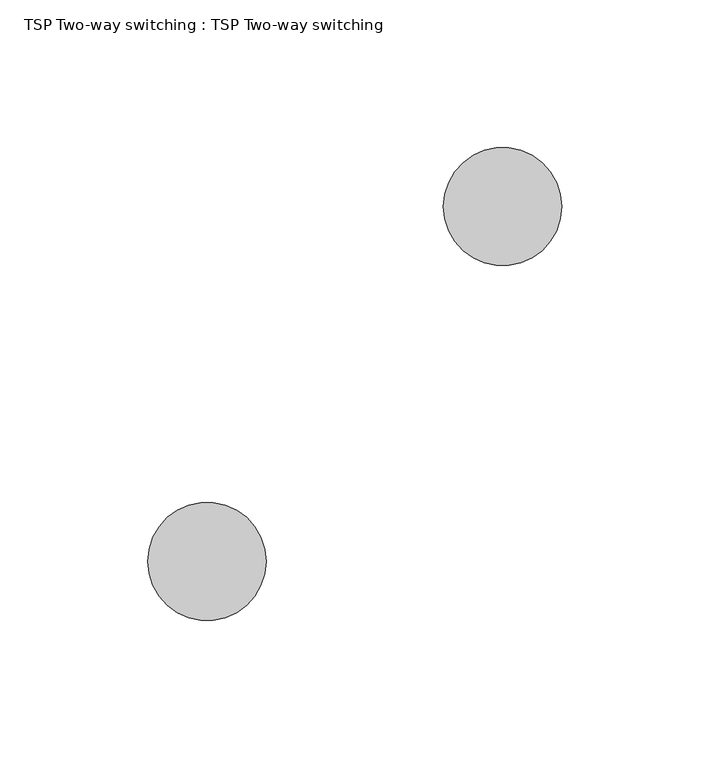
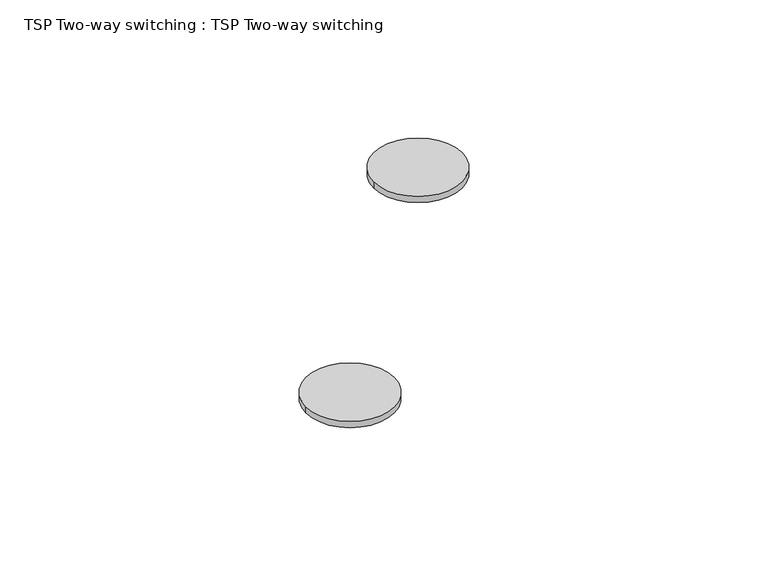
"""IFC4 building model written with IfcOpenShell, lengths in millimetres: proxy geometry, TSP Two-way switching : TSP Two-way switching."""

from ifc_helpers import new_model, si_unit, point, frame_2d, origin, origin_with_axes, place, context, project, spatial, circle_curve, trimmed, segment, composite_curve, outline, extrude, source, transform, mapped, element, save


def tsp_two_way_switching_tsp_two_way_switching_6e80ef18(model_context):
    return source(origin(), model_context, "Body", "SweptSolid", [
        extrude(outline(composite_curve([segment(trimmed(circle_curve(frame_2d((50.0, 60.0)), 20.0), [point((70.0, 60.0))], [point((30.0, 60.0))], False, "CARTESIAN"), True, "CONTINUOUS"), segment(trimmed(circle_curve(frame_2d((50.0, 60.0)), 20.0), [point((30.0, 60.0))], [point((70.0, 60.0))], False, "CARTESIAN"), True, "CONTINUOUS")], self_intersect=False)), origin_with_axes(), (0.0, 0.0, 1.0), 3.0),
        extrude(outline(composite_curve([segment(trimmed(circle_curve(frame_2d((-50.0, -60.0)), 20.0), [point((-70.0, -60.0))], [point((-30.0, -60.0))], False, "CARTESIAN"), True, "CONTINUOUS"), segment(trimmed(circle_curve(frame_2d((-50.0, -60.0)), 20.0), [point((-30.0, -60.0))], [point((-70.0, -60.0))], False, "CARTESIAN"), True, "CONTINUOUS")], self_intersect=False)), origin_with_axes(), (0.0, 0.0, 1.0), 3.0),
    ])


if __name__ == "__main__":
    model = new_model("IFC4")
    model_context = context("Model", 3, world=origin())
    ifc_project = project(units=[si_unit("LENGTHUNIT", "METRE", prefix="MILLI")], contexts=[model_context])
    site = spatial("IfcSite", under=ifc_project)
    building = spatial("IfcBuilding", under=site)
    placement = place(None, origin())
    tsp_two_way_switching_tsp_two_way_switching_shape = tsp_two_way_switching_tsp_two_way_switching_6e80ef18(model_context)
    element("IfcBuildingElementProxy", 1, Name="TSP Two-way switching : TSP Two-way switching", ObjectType="TSP Two-way switching : TSP Two-way switching", at=placement, inside=building, context=model_context, shape_type="MappedRepresentation", body=[
        mapped(tsp_two_way_switching_tsp_two_way_switching_shape, transform((0.0, 0.0, 0.0), x_axis=(1.0, 0.0, 0.0), y_axis=(0.0, 1.0, 0.0), z_axis=(0.0, 0.0, 1.0))),
    ])
    save(model, "model.ifc")

# Revit data of these elements
# Type "TSP Two-way switching : TSP Two-way switching"
#   Model = "TSP_ELEC2WS"
#   Default Elevation = 0
# Element 1 (IfcBuildingElementProxy, "TSP Two-way switching : TSP Two-way switching")
#   Materials on its faces: "Plastic, Opaque Black"
# Materials
#   "Plastic, Opaque Black": class "Plastic", colour RGB 0 0 0, transparency 0.7, Description = "Plastic, generic, opaque black", Cost = 0
